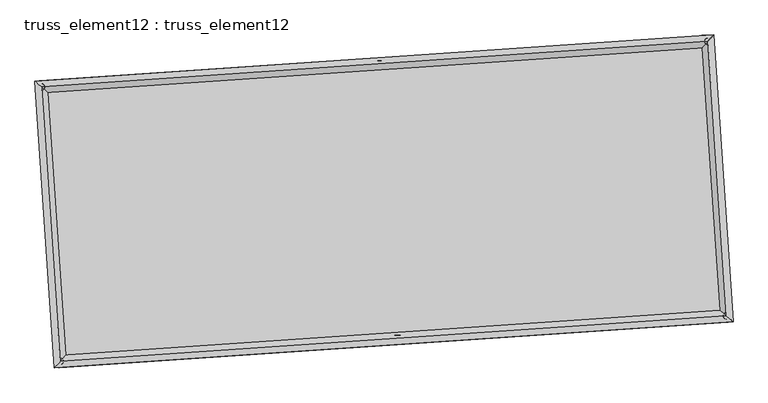
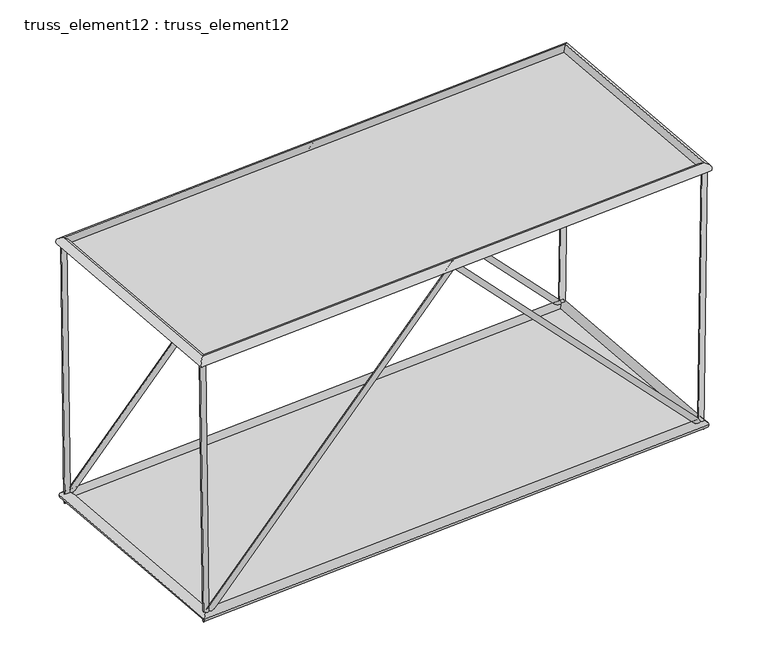
"""IFC4 building model written with IfcOpenShell, lengths in millimetres: plate geometry, truss_element12 : truss_element12."""

from ifc_helpers import new_model, si_unit, frame, origin, origin_with_axes, place, context, project, spatial, polyline, circle_curve, ellipse_curve, outline, extrude, source, transform, mapped, element, save
from ifc_brep_helpers import plane_surface, cylinder_surface, advanced_brep


def truss_element12_truss_element12_bcb7a4b1(model_context):
    return source(origin(), model_context, "Body", "SolidModel", [
        advanced_brep(
        [(-3730.6890845, 2271.7408984, 5000.2232822), (-3829.7838055, 2258.3802507, 4998.9082325), (-3666.5483804, 2276.1144092, 122.5077786), (-3762.4385024, 2262.9722709, -122.5077786), (1064.3227767, 2598.6945297, 5071.6784045), (1064.7619686, 2592.1207211, 4927.4371435), (5794.0163085, 2921.1943524, 122.4994051), (5890.7446685, 2921.1861361, -122.4994051), (5859.3257876, 2925.6475575, 5000.2192941), (5959.316593, 2925.861795, 4998.880287)],
        [
            (0, 1, circle_curve(frame((-3780.236445, 2265.0605745, 4999.5657574), z_axis=(-0.013148600710356454, -0.000896553099930443, 0.9999131514746162), x_axis=(-0.13360666404585098, 0.9910340586353044, -0.0008683014310743792)), 50.0)),
            (1, 0, circle_curve(frame((-3780.236445, 2265.0605745, 4999.5657574), z_axis=(-0.013148600710356454, -0.000896553099930443, 0.9999131514746162), x_axis=(-0.13360666404585098, 0.9910340586353044, -0.0008683014310743792)), 50.0)),
            (0, 2),
            (2, 3, ellipse_curve(frame((-3714.4934414, 2269.54334, 0.0), z_axis=(-0.928200365252963, -0.06329045448668467, 0.3666584245795189), x_axis=(0.3658090222339585, 0.024943126655854568, 0.93035563075894)), 131.9651677, 50.0)),
            (3, 1),
            (3, 2, ellipse_curve(frame((-3714.4934414, 2269.54334, 0.0), z_axis=(-0.928200365252963, -0.06329045448668467, 0.3666584245795189), x_axis=(0.3658090222339585, 0.024943126655854568, 0.93035563075894)), 131.9651677, 50.0)),
            (2, 4),
            (4, 5, ellipse_curve(frame((1064.5423727, 2595.4076254, 4999.557774), z_axis=(-0.9976833941197889, -0.06802823809539234, 6.260394869410126e-05), x_axis=(-6.245892014097819e-05, -4.258836334217303e-06, -0.9999999980403728)), 72.2776719, 50.0)),
            (5, 3),
            (5, 4, ellipse_curve(frame((1064.5423727, 2595.4076254, 4999.557774), z_axis=(-0.9976833941197889, -0.06802823809539234, 6.260394869410126e-05), x_axis=(-6.245892014097819e-05, -4.258836334217303e-06, -0.9999999980403728)), 72.2776719, 50.0)),
            (4, 6),
            (6, 7, ellipse_curve(frame((5842.3804885, 2921.1902443, 0.0), z_axis=(-0.9282671693555778, -0.06329500960449407, -0.3664884773846918), x_axis=(-0.36563946873947, -0.02493156544760182, 0.930422589979548)), 131.9466513, 50.0)),
            (7, 5),
            (7, 6, ellipse_curve(frame((5842.3804885, 2921.1902443, 0.0), z_axis=(-0.9282671693555778, -0.06329500960449407, -0.3664884773846918), x_axis=(-0.36563946873947, -0.02493156544760182, 0.930422589979548)), 131.9466513, 50.0)),
            (8, 9, circle_curve(frame((5909.3211903, 2925.7546762, 4999.5497906), z_axis=(0.013388140355829114, 0.0009128863977761105, 0.9999099581143482), x_axis=(-0.002154405773521634, 0.9999972884300797, -0.0008841200433773456)), 50.0)),
            (9, 8, circle_curve(frame((5909.3211903, 2925.7546762, 4999.5497906), z_axis=(0.013388140355829114, 0.0009128863977761105, 0.9999099581143482), x_axis=(-0.002154405773521634, 0.9999972884300797, -0.0008841200433773456)), 50.0)),
            (6, 8),
            (9, 7),
        ],
        [
            plane_surface(frame((-3780.236445, 2315.0605545, 4999.6105889), z_axis=(-0.01314860071035555, -0.000896553099925358, 0.9999131514746165), x_axis=(0.9999135534131738, -1.1789437883713555e-05, 0.01314859542496904))),
            cylinder_surface(frame((-3780.236445, 2265.0605745, 4999.5657574), z_axis=(-0.01314860071035645, -0.0008965530999304427, 0.999913151474616), x_axis=(-0.13360666404585098, 0.9910340586353044, -0.0008683014310743792)), 50.0),
            cylinder_surface(frame((-3714.4934414, 2269.54334, 0.0), z_axis=(-0.6902190995054774, -0.04706341662684533, -0.7220682997426603), x_axis=(-0.02041747777222218, 0.9987519989749245, -0.045580381141596744)), 50.0),
            cylinder_surface(frame((1064.5423727, 2595.4076254, 4999.557774), z_axis=(-0.6901288948828257, -0.04705726591652891, 0.7221549156325607), x_axis=(-0.11534907557209756, 0.9922789741897385, -0.045574424248946074)), 50.0),
            plane_surface(frame((5909.3211903, 2875.7546971, 4999.595439), z_axis=(0.01338814035582826, 0.000912886397775815, 0.9999099581143482), x_axis=(0.9999103748325711, -1.2222946706330628e-05, -0.013388134776246131))),
            cylinder_surface(frame((5842.3804885, 2921.1902443, 0.0), z_axis=(-0.013388140355829114, -0.0009128863977761105, -0.9999099581143482), x_axis=(-0.002154405773521634, 0.9999972884300797, -0.0008841200433773456)), 50.0),
        ],
        [
            (0, [[1, 2]]),
            (1, [[-1, 3, 4, 5]]),
            (1, [[-2, -5, 6, -3]]),
            (2, [[-4, 7, 8, 9]]),
            (2, [[-6, -9, 10, -7]]),
            (3, [[-8, 11, 12, 13]]),
            (3, [[-10, -13, 14, -11]]),
            (4, [[15, 16]]),
            (5, [[-12, 17, -16, 18]]),
            (5, [[-14, -18, -15, -17]]),
        ],
    ),
        advanced_brep(
        [(-3458.5761315, -1718.9926859, 5000.2232822), (-3557.6708526, -1732.3533336, 4998.9082325), (-3394.4354275, -1714.6191751, 122.5077786), (-3490.3255495, -1727.7613134, -122.5077786), (1336.4357296, -1392.0390546, 5071.6784045), (1336.8749216, -1398.6128632, 4927.4371435), (6066.1292614, -1069.5392319, 122.4994051), (6162.8576214, -1069.5474482, -122.4994051), (6131.4387405, -1065.0860268, 5000.2192941), (6231.4295459, -1064.8717893, 4998.880287)],
        [
            (0, 1, circle_curve(frame((-3508.1234921, -1725.6730098, 4999.5657574), z_axis=(-0.013148600710356402, -0.0008965530999304543, 0.9999131514746161), x_axis=(-0.13360666404585028, 0.9910340586353045, -0.0008683014310743518)), 50.0)),
            (1, 0, circle_curve(frame((-3508.1234921, -1725.6730098, 4999.5657574), z_axis=(-0.013148600710356402, -0.0008965530999304543, 0.9999131514746161), x_axis=(-0.13360666404585028, 0.9910340586353045, -0.0008683014310743518)), 50.0)),
            (0, 2),
            (2, 3, ellipse_curve(frame((-3442.3804885, -1721.1902443, 0.0), z_axis=(-0.928200365252963, -0.06329045448668438, 0.36665842457951897), x_axis=(0.36580902223395856, 0.024943126655854433, 0.9303556307589399)), 131.9651677, 50.0)),
            (3, 1),
            (3, 2, ellipse_curve(frame((-3442.3804885, -1721.1902443, 0.0), z_axis=(-0.928200365252963, -0.06329045448668438, 0.36665842457951897), x_axis=(0.36580902223395856, 0.024943126655854433, 0.9303556307589399)), 131.9651677, 50.0)),
            (2, 4),
            (4, 5, ellipse_curve(frame((1336.6553256, -1395.3259589, 4999.557774), z_axis=(-0.997683394119789, -0.06802823809539227, 6.260394869466301e-05), x_axis=(-6.245892014143939e-05, -4.258836333986682e-06, -0.9999999980403728)), 72.2776719, 50.0)),
            (5, 3),
            (5, 4, ellipse_curve(frame((1336.6553256, -1395.3259589, 4999.557774), z_axis=(-0.997683394119789, -0.06802823809539227, 6.260394869466301e-05), x_axis=(-6.245892014143939e-05, -4.258836333986682e-06, -0.9999999980403728)), 72.2776719, 50.0)),
            (4, 6),
            (6, 7, ellipse_curve(frame((6114.4934414, -1069.54334, 0.0), z_axis=(-0.9282671693555782, -0.06329500960449432, -0.36648847738469165), x_axis=(-0.3656394687394694, -0.02493156544760184, 0.9304225899795483)), 131.9466513, 50.0)),
            (7, 5),
            (7, 6, ellipse_curve(frame((6114.4934414, -1069.54334, 0.0), z_axis=(-0.9282671693555782, -0.06329500960449432, -0.36648847738469165), x_axis=(-0.3656394687394694, -0.02493156544760184, 0.9304225899795483)), 131.9466513, 50.0)),
            (8, 9, circle_curve(frame((6181.4341432, -1064.9789081, 4999.5497906), z_axis=(0.013388140355828559, 0.0009128863977761051, 0.9999099581143482), x_axis=(-0.0021544057735223424, 0.9999972884300797, -0.0008841200433773321)), 50.0)),
            (9, 8, circle_curve(frame((6181.4341432, -1064.9789081, 4999.5497906), z_axis=(0.013388140355828559, 0.0009128863977761051, 0.9999099581143482), x_axis=(-0.0021544057735223424, 0.9999972884300797, -0.0008841200433773321)), 50.0)),
            (6, 8),
            (9, 7),
        ],
        [
            plane_surface(frame((-3508.1234921, -1675.6730298, 4999.6105889), z_axis=(-0.01314860071035555, -0.0008965530999253677, 0.9999131514746165), x_axis=(0.9999135534131738, -1.1789437883713555e-05, 0.01314859542496904))),
            cylinder_surface(frame((-3508.1234921, -1725.6730098, 4999.5657574), z_axis=(-0.013148600710356402, -0.0008965530999304543, 0.9999131514746161), x_axis=(-0.13360666404585028, 0.9910340586353045, -0.0008683014310743518)), 50.0),
            cylinder_surface(frame((-3442.3804885, -1721.1902443, 0.0), z_axis=(-0.6902190995054773, -0.04706341662684507, -0.7220682997426601), x_axis=(-0.020417477772222078, 0.9987519989749246, -0.0455803811415965)), 50.0),
            cylinder_surface(frame((1336.6553256, -1395.3259589, 4999.557774), z_axis=(-0.6901288948828249, -0.04705726591652899, 0.7221549156325613), x_axis=(-0.11534907557209753, 0.9922789741897384, -0.045574424248945776)), 50.0),
            plane_surface(frame((6181.4341432, -1114.9788872, 4999.595439), z_axis=(0.013388140355828259, 0.0009128863977758237, 0.9999099581143482), x_axis=(0.9999103748325711, -1.2222946705886538e-05, -0.013388134776246131))),
            cylinder_surface(frame((6114.4934414, -1069.54334, 0.0), z_axis=(-0.013388140355828559, -0.0009128863977761051, -0.9999099581143482), x_axis=(-0.0021544057735223424, 0.9999972884300797, -0.0008841200433773321)), 50.0),
        ],
        [
            (0, [[1, 2]]),
            (1, [[-1, 3, 4, 5]]),
            (1, [[-2, -5, 6, -3]]),
            (2, [[-4, 7, 8, 9]]),
            (2, [[-6, -9, 10, -7]]),
            (3, [[-8, 11, 12, 13]]),
            (3, [[-10, -13, 14, -11]]),
            (4, [[15, 16]]),
            (5, [[-12, 17, -16, 18]]),
            (5, [[-14, -18, -15, -17]]),
        ],
    ),
        advanced_brep(
        [(-3508.127679, -1725.6776503, 4909.5657575), (-3508.1193051, -1725.6683692, 5089.5657573), (-3780.2316669, 2265.0565453, 5089.5657573), (-3780.2412231, 2265.0646038, 4909.5657575), (5909.3172986, 2925.7500558, 5089.5497905), (5909.325082, 2925.7592967, 4909.5497907), (6181.4296603, -1064.9748587, 5089.5497905), (6181.4386261, -1064.9829574, 4909.5497907)],
        [
            (0, 1, ellipse_curve(frame((-3508.1234921, -1725.6730098, 4999.5657574), z_axis=(-0.7535719234045049, 0.6573654662781456, 1.1624966694194113e-06), x_axis=(-0.6573654662771273, -0.753571923405393, 1.1624966755451343e-06)), 127.2792206, 90.0)),
            (1, 2),
            (2, 3, ellipse_curve(frame((-3780.236445, 2265.0605745, 4999.5657574), z_axis=(-0.6573654662771272, -0.753571923405393, 1.1624966742049372e-06), x_axis=(0.7535719234045045, -0.6573654662781458, -1.162496668079214e-06)), 127.2792206, 90.0)),
            (3, 0),
            (1, 0, ellipse_curve(frame((-3508.1234921, -1725.6730098, 4999.5657574), z_axis=(-0.7535719234045049, 0.6573654662781456, 1.1624966694194113e-06), x_axis=(-0.6573654662771273, -0.753571923405393, 1.1624966755451343e-06)), 127.2792206, 90.0)),
            (3, 2, ellipse_curve(frame((-3780.236445, 2265.0605745, 4999.5657574), z_axis=(-0.6573654662771272, -0.753571923405393, 1.1624966742049372e-06), x_axis=(0.7535719234045045, -0.6573654662781458, -1.162496668079214e-06)), 127.2792206, 90.0)),
            (2, 4),
            (4, 5, ellipse_curve(frame((5909.3211903, 2925.7546762, 4999.5497906), z_axis=(-0.7535719234045039, 0.6573654662781465, 1.1624966713335448e-06), x_axis=(-0.6573654662771284, -0.7535719234053921, 1.1624966709506072e-06)), 127.2792206, 90.0)),
            (5, 3),
            (5, 4, ellipse_curve(frame((5909.3211903, 2925.7546762, 4999.5497906), z_axis=(-0.7535719234045039, 0.6573654662781465, 1.1624966713335448e-06), x_axis=(-0.6573654662771284, -0.7535719234053921, 1.1624966709506072e-06)), 127.2792206, 90.0)),
            (4, 6),
            (6, 7, ellipse_curve(frame((6181.4341432, -1064.9789081, 4999.5497906), z_axis=(0.6573654662771281, 0.7535719234053923, -1.1624966722908037e-06), x_axis=(-0.7535719234045039, 0.6573654662781466, 1.1624966726737413e-06)), 127.2792206, 90.0)),
            (7, 5),
            (7, 6, ellipse_curve(frame((6181.4341432, -1064.9789081, 4999.5497906), z_axis=(0.6573654662771281, 0.7535719234053923, -1.1624966722908037e-06), x_axis=(-0.7535719234045039, 0.6573654662781466, 1.1624966726737413e-06)), 127.2792206, 90.0)),
            (6, 1),
            (0, 7),
        ],
        [
            cylinder_surface(frame((-3508.1234921, -1725.6730098, 4999.5657574), z_axis=(0.06802823822870312, -0.9976833960748764, 0.0), x_axis=(-0.9976833948316876, -0.0680282381439348, 4.9921449588598364e-05)), 90.0),
            cylinder_surface(frame((-3780.236445, 2265.0605745, 4999.5657574), z_axis=(-0.9976833960735286, -0.06802823822860814, 1.6440185585427e-06), x_axis=(-0.06802823807023788, 0.9976833949176206, 4.8277431027640126e-05)), 90.0),
            cylinder_surface(frame((5909.3211903, 2925.7546762, 4999.5497906), z_axis=(-0.0680282382287005, 0.9976833960748769, 0.0), x_axis=(0.9976833949900581, 0.06802823815473083, 4.663341247074265e-05)), 90.0),
            cylinder_surface(frame((6181.4341432, -1064.9789081, 4999.5497906), z_axis=(0.9976833960735284, 0.06802823822860798, -1.6440185604380239e-06), x_axis=(0.06802823822860797, -0.9976833949068218, 4.8277431028994146e-05)), 90.0),
        ],
        [
            (0, [[1, 2, 3, 4]]),
            (0, [[5, -4, 6, -2]]),
            (1, [[-3, 7, 8, 9]]),
            (1, [[-6, -9, 10, -7]]),
            (2, [[-8, 11, 12, 13]]),
            (2, [[-10, -13, 14, -11]]),
            (3, [[-12, 15, -1, 16]]),
            (3, [[-14, -16, -5, -15]]),
        ],
    ),
        advanced_brep(
        [(-3358.7115243, -1625.2761972, 0.0), (-3526.0494527, -1817.1042913, 0.0), (-3810.4074885, 2353.2123043, 0.0), (-3618.5793943, 2185.8743758, 0.0), (5926.0494527, 3017.1042913, 0.0), (5758.7115243, 2825.2761972, 0.0), (6210.4074885, -1153.2123043, 0.0), (6018.5793943, -985.8743758, 0.0)],
        [
            (0, 1, ellipse_curve(frame((-3442.3804885, -1721.1902443, 0.0), z_axis=(-0.7535719234054598, 0.6573654662780787, 0.0), x_axis=(-0.6573654662780786, -0.7535719234054599, 0.0)), 127.2792206, 90.0)),
            (1, 2),
            (2, 3, ellipse_curve(frame((-3714.4934414, 2269.54334, 0.0), z_axis=(-0.6573654662780787, -0.7535719234054596, 0.0), x_axis=(0.7535719234054594, -0.657365466278079, 0.0)), 127.2792206, 90.0)),
            (3, 0),
            (1, 0, ellipse_curve(frame((-3442.3804885, -1721.1902443, 0.0), z_axis=(-0.7535719234054598, 0.6573654662780787, 0.0), x_axis=(-0.6573654662780786, -0.7535719234054599, 0.0)), 127.2792206, 90.0)),
            (3, 2, ellipse_curve(frame((-3714.4934414, 2269.54334, 0.0), z_axis=(-0.6573654662780787, -0.7535719234054596, 0.0), x_axis=(0.7535719234054594, -0.657365466278079, 0.0)), 127.2792206, 90.0)),
            (2, 4),
            (4, 5, ellipse_curve(frame((5842.3804885, 2921.1902443, 0.0), z_axis=(-0.7535719234054591, 0.6573654662780796, 0.0), x_axis=(-0.6573654662780795, -0.753571923405459, 0.0)), 127.2792206, 90.0)),
            (5, 3),
            (5, 4, ellipse_curve(frame((5842.3804885, 2921.1902443, 0.0), z_axis=(-0.7535719234054591, 0.6573654662780796, 0.0), x_axis=(-0.6573654662780795, -0.753571923405459, 0.0)), 127.2792206, 90.0)),
            (4, 6),
            (6, 7, ellipse_curve(frame((6114.4934414, -1069.54334, 0.0), z_axis=(0.6573654662780797, 0.7535719234054589, 0.0), x_axis=(-0.7535719234054589, 0.6573654662780799, 0.0)), 127.2792206, 90.0)),
            (7, 5),
            (7, 6, ellipse_curve(frame((6114.4934414, -1069.54334, 0.0), z_axis=(0.6573654662780797, 0.7535719234054589, 0.0), x_axis=(-0.7535719234054589, 0.6573654662780799, 0.0)), 127.2792206, 90.0)),
            (6, 1),
            (0, 7),
        ],
        [
            cylinder_surface(frame((-3442.3804885, -1721.1902443, 0.0), z_axis=(0.06802823822870559, -0.9976833960748764, 0.0), x_axis=(-0.9976833960748764, -0.06802823822870559, 0.0)), 90.0),
            cylinder_surface(frame((-3714.4934414, 2269.54334, 0.0), z_axis=(-0.9976833960748767, -0.06802823822870269, 0.0), x_axis=(-0.06802823822870269, 0.9976833960748767, 0.0)), 90.0),
            cylinder_surface(frame((5842.3804885, 2921.1902443, 0.0), z_axis=(-0.068028238228703, 0.9976833960748764, 0.0), x_axis=(0.9976833960748764, 0.068028238228703, 0.0)), 90.0),
            cylinder_surface(frame((6114.4934414, -1069.54334, 0.0), z_axis=(0.9976833960748765, 0.06802823822870231, 0.0), x_axis=(0.06802823822870231, -0.9976833960748765, 0.0)), 90.0),
        ],
        [
            (0, [[1, 2, 3, 4]]),
            (0, [[5, -4, 6, -2]]),
            (1, [[-3, 7, 8, 9]]),
            (1, [[-6, -9, 10, -7]]),
            (2, [[-8, 11, 12, 13]]),
            (2, [[-10, -13, 14, -11]]),
            (3, [[-12, 15, -1, 16]]),
            (3, [[-14, -16, -5, -15]]),
        ],
    ),
        extrude(outline(polyline([(-3442.3804885, -1721.1902443), (-3714.4934414, 2269.54334), (5842.3804885, 2921.1902443), (6114.4934414, -1069.54334), (-3442.3804885, -1721.1902443)])), origin_with_axes(), (0.0, 0.0, 1.0), 20.0),
        extrude(outline(polyline([(-2000.0, 4856.0283119), (2000.0, 4856.0283119), (2000.0, -4856.0283119), (-2000.0, -4856.0283119), (-2000.0, 4856.0283119)])), frame((1200.5988491, 600.0408332, 4999.557774), z_axis=(1.6402100184022758e-06, 1.1183969047438534e-07, 0.9999999999986487), x_axis=(-0.06802823822870536, 0.9976833960748763, 0.0)), (0.0, 0.0, 1.0), 20.0),
    ])


if __name__ == "__main__":
    model = new_model("IFC4")
    model_context = context("Model", 3, world=origin())
    ifc_project = project(units=[si_unit("LENGTHUNIT", "METRE", prefix="MILLI")], contexts=[model_context])
    site = spatial("IfcSite", under=ifc_project)
    building = spatial("IfcBuilding", under=site)
    placement = place(None, origin())
    truss_element12_truss_element12_shape = truss_element12_truss_element12_bcb7a4b1(model_context)
    element("IfcPlate", 1, ObjectType="truss_element12 : truss_element12", at=placement, inside=building, context=model_context, shape_type="MappedRepresentation", body=[
        mapped(truss_element12_truss_element12_shape, transform((0.0, 0.0, 0.0), x_axis=(1.0, 0.0, 0.0), y_axis=(0.0, 1.0, 0.0), z_axis=(0.0, 0.0, 1.0))),
    ])
    save(model, "model.ifc")

# Revit data of these elements
# Type "truss_element12 : truss_element12"
#   steellbar1 = 90 mm
#   steelbar2 = 50 mm
#   offset1 = 5000 mm
#   M = Default Roof
# Element 1 (IfcPlate, "truss_element12 : truss_element12")
#   Materials on its faces: "Default Roof"
# Materials
#   "Default Roof": class "Miscellaneous", colour RGB 0 127 0, transparency 0, Comments = "Rendering appearance not upgraded Rendering appearance not upgraded ", Cost = 0
